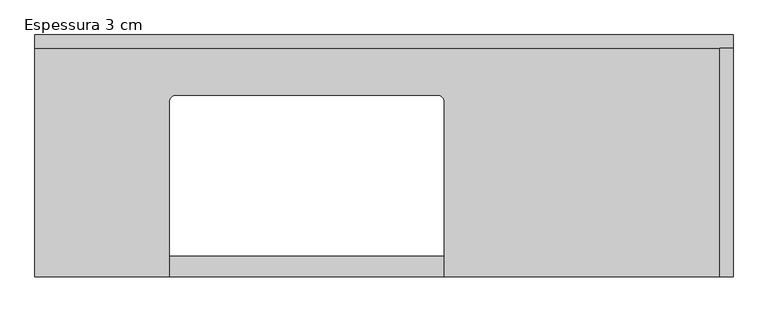
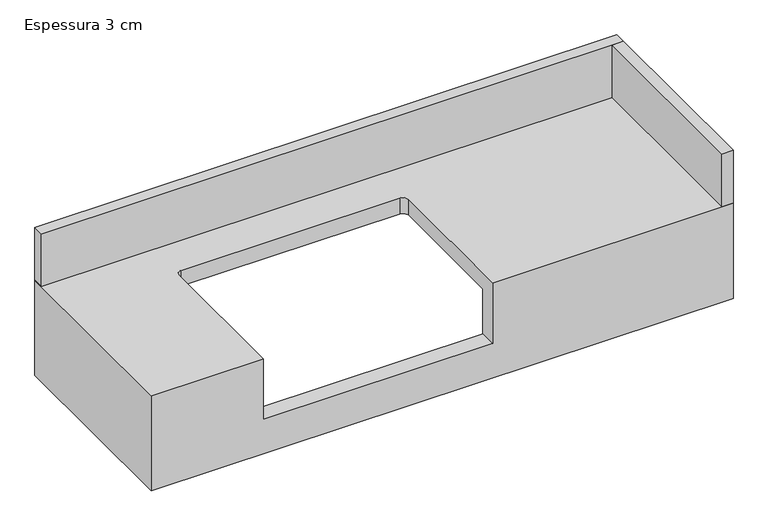
"""IFC4 building model written with IfcOpenShell, lengths in millimetres: furniture geometry, CC_BANCADA BANHEIRO COM CUBA_CANTO RETO : Espessura 3 cm."""

from ifc_helpers import new_model, si_unit, frame, origin, place, context, project, spatial, polyline, circle_curve, outline, extrude, source, transform, mapped, element, save
from ifc_brep_helpers import plane_surface, revolved_surface, advanced_brep


def espessura_3_cm_1ecb3cbd(model_context):
    return source(origin(), model_context, "Body", "SolidModel", [
        advanced_brep(
        [(750.0, 300.0, 860.0), (-290.0, 300.0, 860.0), (-290.0, -60.0, 860.0), (-90.0, -60.0, 860.0), (-90.0, 200.0, 860.0), (-80.0, 210.0, 860.0), (310.0, 210.0, 860.0), (320.0, 200.0, 860.0), (320.0, -60.0, 860.0), (750.0, -60.0, 860.0), (750.0, 300.0, 680.0), (720.0, 300.0, 680.0), (720.0, 300.0, 830.0), (-260.0, 300.0, 830.0), (-260.0, 300.0, 680.0), (-290.0, 300.0, 680.0), (-290.0, -60.0, 680.0), (750.0, -60.0, 680.0), (320.0, -60.0, 745.0), (-90.0, -60.0, 745.0), (720.0, -30.0, 830.0), (320.0, -30.0, 830.0), (320.0, 200.0, 830.0), (310.0, 210.0, 830.0), (-80.0, 210.0, 830.0), (-90.0, 200.0, 830.0), (-90.0, -30.0, 830.0), (-260.0, -30.0, 830.0), (-260.0, -30.0, 680.0), (-90.0, -30.0, 745.0), (320.0, -30.0, 745.0), (720.0, -30.0, 680.0)],
        [
            (0, 1),
            (1, 2),
            (2, 3),
            (3, 4),
            (4, 5, circle_curve(frame((-80.0, 200.0, 860.0), z_axis=(0.0, 0.0, -1.0), x_axis=(0.0, 1.0, 0.0)), 10.0)),
            (5, 6),
            (6, 7, circle_curve(frame((310.0, 200.0, 860.0), z_axis=(0.0, 0.0, -1.0), x_axis=(0.0, 1.0, 0.0)), 10.0)),
            (7, 8),
            (8, 9),
            (9, 0),
            (0, 10),
            (10, 11),
            (11, 12),
            (12, 13),
            (13, 14),
            (14, 15),
            (15, 1),
            (15, 16),
            (16, 2),
            (16, 17),
            (17, 9),
            (8, 18),
            (18, 19),
            (19, 3),
            (17, 10),
            (12, 20),
            (20, 21),
            (21, 22),
            (22, 23, circle_curve(frame((310.0, 200.0, 830.0), z_axis=(0.0, 0.0, 1.0), x_axis=(0.0, 1.0, 0.0)), 10.0)),
            (23, 24),
            (24, 25, circle_curve(frame((-80.0, 200.0, 830.0), z_axis=(0.0, 0.0, 1.0), x_axis=(0.0, 1.0, 0.0)), 10.0)),
            (25, 26),
            (26, 27),
            (27, 13),
            (27, 28),
            (28, 14),
            (26, 29),
            (29, 30),
            (30, 21),
            (20, 31),
            (31, 28),
            (11, 31),
            (5, 24),
            (23, 6),
            (18, 30),
            (29, 19),
            (4, 25),
            (7, 22),
        ],
        [
            plane_surface(frame((-290.0, 300.0, 860.0), z_axis=(0.0, 0.0, 1.0), x_axis=(-1.0, 0.0, 0.0))),
            plane_surface(frame((750.0, 300.0, 860.0), z_axis=(0.0, 1.0, 0.0), x_axis=(0.0, 0.0, -1.0))),
            plane_surface(frame((-290.0, 300.0, 860.0), z_axis=(-1.0, 0.0, 0.0), x_axis=(0.0, 0.0, -1.0))),
            plane_surface(frame((-290.0, -60.0, 860.0), z_axis=(0.0, -1.0, 0.0), x_axis=(0.0, 0.0, -1.0))),
            plane_surface(frame((750.0, -60.0, 860.0), z_axis=(1.0, 0.0, 0.0), x_axis=(0.0, 0.0, -1.0))),
            plane_surface(frame((-260.0, 300.0, 830.0), z_axis=(0.0, 0.0, -1.0), x_axis=(-1.0, 0.0, 0.0))),
            plane_surface(frame((-260.0, 300.0, 830.0), z_axis=(1.0, 0.0, 0.0), x_axis=(0.0, 0.0, -1.0))),
            plane_surface(frame((-260.0, -30.0, 830.0), z_axis=(0.0, 1.0, 0.0), x_axis=(0.0, 0.0, -1.0))),
            plane_surface(frame((720.0, -30.0, 830.0), z_axis=(-1.0, 0.0, 0.0), x_axis=(0.0, 0.0, -1.0))),
            plane_surface(frame((750.0, -60.0, 680.0), z_axis=(0.0, 0.0, -1.0), x_axis=(0.0, 1.0, 0.0))),
            plane_surface(frame((-80.0, 210.0, 745.0), z_axis=(0.0, -1.0, 0.0), x_axis=(0.0, 0.0, 1.0))),
            plane_surface(frame((310.0, 210.0, 745.0), z_axis=(0.0, 0.0, 1.0), x_axis=(1.0, 0.0, 0.0))),
            revolved_surface(polyline([(-80.0, 210.0, 830.0), (-80.0, 210.0, 860.0)]), (-80.0, 200.0, 900.0), (0.0, 0.0, -1.0)),
            plane_surface(frame((-90.0, -190.0, 745.0), z_axis=(1.0, 0.0, 0.0), x_axis=(0.0, 0.0, 1.0))),
            plane_surface(frame((320.0, 200.0, 745.0), z_axis=(-1.0, 0.0, 0.0), x_axis=(0.0, 0.0, 1.0))),
            revolved_surface(polyline([(310.0, 210.0, 830.0), (310.0, 210.0, 860.0)]), (310.0, 200.0, 900.0), (0.0, 0.0, -1.0)),
        ],
        [
            (0, [[1, 2, 3, 4, 5, 6, 7, 8, 9, 10]]),
            (1, [[-1, 11, 12, 13, 14, 15, 16, 17]]),
            (2, [[-2, -17, 18, 19]]),
            (3, [[-3, -19, 20, 21, -9, 22, 23, 24]]),
            (4, [[-10, -21, 25, -11]]),
            (5, [[26, 27, 28, 29, 30, 31, 32, 33, 34, -14]]),
            (6, [[-34, 35, 36, -15]]),
            (7, [[-33, 37, 38, 39, -27, 40, 41, -35]]),
            (8, [[-26, -13, 42, -40]]),
            (9, [[-12, -25, -20, -18, -16, -36, -41, -42]]),
            (10, [[-6, 43, -30, 44]]),
            (11, [[-23, 45, -38, 46]]),
            (12, [[-5, 47, -31, -43]]),
            (13, [[-4, -24, -46, -37, -32, -47]]),
            (14, [[-8, 48, -28, -39, -45, -22]]),
            (15, [[-7, -44, -29, -48]]),
        ],
    ),
        extrude(outline(polyline([(730.0, 280.0), (750.0, 280.0), (750.0, -60.0), (730.0, -60.0), (730.0, 280.0)])), frame((0.0, 0.0, 860.0), z_axis=(0.0, 0.0, 1.0), x_axis=(1.0, 0.0, 0.0)), (0.0, 0.0, 1.0), 100.0),
        extrude(outline(polyline([(750.0, 300.0), (750.0, 280.0), (-290.0, 280.0), (-290.0, 300.0), (750.0, 300.0)])), frame((0.0, 0.0, 860.0), z_axis=(0.0, 0.0, 1.0), x_axis=(1.0, 0.0, 0.0)), (0.0, 0.0, 1.0), 100.0),
    ])


if __name__ == "__main__":
    model = new_model("IFC4")
    model_context = context("Model", 3, world=origin())
    ifc_project = project(units=[si_unit("LENGTHUNIT", "METRE", prefix="MILLI")], contexts=[model_context])
    site = spatial("IfcSite", under=ifc_project)
    building = spatial("IfcBuilding", under=site)
    placement = place(None, origin())
    espessura_3_cm_shape = espessura_3_cm_1ecb3cbd(model_context)
    element("IfcFurniture", 1, ObjectType="CC_BANCADA BANHEIRO COM CUBA_CANTO RETO : Espessura 3 cm", at=placement, inside=building, context=model_context, shape_type="MappedRepresentation", body=[
        mapped(espessura_3_cm_shape, transform((0.0, 0.0, 0.0), x_axis=(1.0, 0.0, 0.0), y_axis=(0.0, 1.0, 0.0), z_axis=(0.0, 0.0, 1.0))),
    ])
    save(model, "model.ifc")

# Revit data of these elements
# Type "CC_BANCADA BANHEIRO COM CUBA_CANTO RETO : Espessura 3 cm"
#   Uso HS [instance default] = ""
#   h TESTEIRA AUX [instance default] = 0.15 m
#   Altura testeira [instance default] = 0.15 m
#   Altura rodapia [instance default] = 0.10 m
#   Espessura rodapia [instance default] = 0.02 m
#   Prof/2 [instance default] = 0.20 m
#   Offset cuba esquerda [instance default] = 0.40 m
#   Depth [instance default] = 1.20 m
#   Width [instance default] = 0.40 m
#   Espessura bancada = 0.03 m
#   Comprimento [instance default] = 1.20 m
#   Height [instance default] = 0.86 m
#   Testeira [instance default] = yes
#   Rodapia fundo [instance default] = no
#   Rodapia esquerda [instance default] = no
#   Rodapia direita [instance default] = no
#   Material porta-toalha [instance default] = .CROMADO
#   Material hidráulico [instance default] = .CROMADO
#   Material cuba [instance default] = .PORCELANA BRANCA
#   Material bancada [instance default] = .GRANITO_BRANCO_ITAUNAS
#   Assembly Code = ""
# Element 1 (IfcFurniture, "CC_BANCADA BANHEIRO COM CUBA_CANTO RETO : Espessura 3 cm")
#   Uso HS = "VESTIÁRIO"
#   Prof/2 = 0.18 m
#   Offset cuba esquerda = 0.20 m
#   Depth = 1.04 m
#   Width = 0.36 m
#   Comprimento = 1.04 m
#   Rodapia fundo = yes
#   Rodapia direita = yes
#   Materials on its faces: ".GRANITO_BRANCO_ITAUNAS"
# Materials
#   ".CROMADO": class "CC_METAIS", colour RGB 211 223 226, transparency 0, Cost = 0
#   ".PORCELANA BRANCA": class "CC_PORCELANA", colour RGB 230 230 230, transparency 0, Cost = 0
#   ".GRANITO_BRANCO_ITAUNAS": class ".CC_PEDRA REVEST.", colour RGB 202 195 174, transparency 0, Description = "Revestimento em granito", Cost = 0
